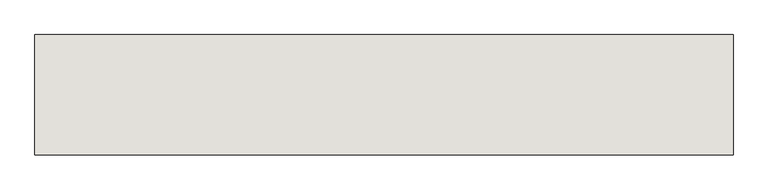
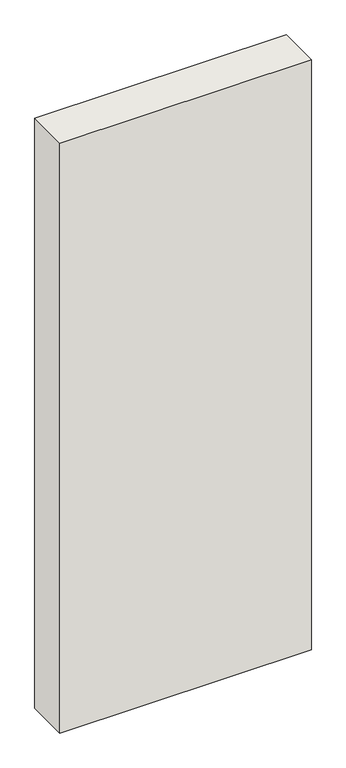
"""IFC4 building model written with IfcOpenShell, lengths in millimetres: wall geometry, Holzwand."""

from ifc_helpers import new_model, si_unit, origin, origin_with_axes, place, context, project, spatial, polyline, outline, extrude, source, transform, mapped, element, save


def wall_6afbbe25(model_context):
    return source(origin(), model_context, "Body", "SweptSolid", [
        extrude(outline(polyline([(0.0, 200.0), (1161.7, 200.0), (1161.7, 0.0), (0.0, 0.0), (0.0, 200.0)])), origin_with_axes(), (0.0, 0.0, 1.0), 2880.0),
    ])


if __name__ == "__main__":
    model = new_model("IFC4")
    model_context = context("Model", 3, world=origin())
    ifc_project = project(units=[si_unit("LENGTHUNIT", "METRE", prefix="MILLI")], contexts=[model_context])
    site = spatial("IfcSite", under=ifc_project)
    building = spatial("IfcBuilding", under=site)
    placement = place(None, origin())
    wall_shape = wall_6afbbe25(model_context)
    element("IfcWall", 1, ObjectType="Holzwand", at=placement, inside=building, context=model_context, shape_type="MappedRepresentation", body=[
        mapped(wall_shape, transform((0.0, 0.0, 0.0), x_axis=(1.0, 0.0, 0.0), y_axis=(0.0, 1.0, 0.0), z_axis=(0.0, 0.0, 1.0))),
    ])
    save(model, "model.ifc")

# Revit data of these elements
# Element 1 (IfcWall, "Holzwand")
#   Materials on its faces: "holzschalung"
# Materials
#   "holzschalung": class "Unassigned", colour RGB 128 128 128, transparency 0
